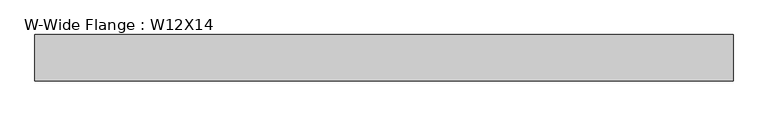
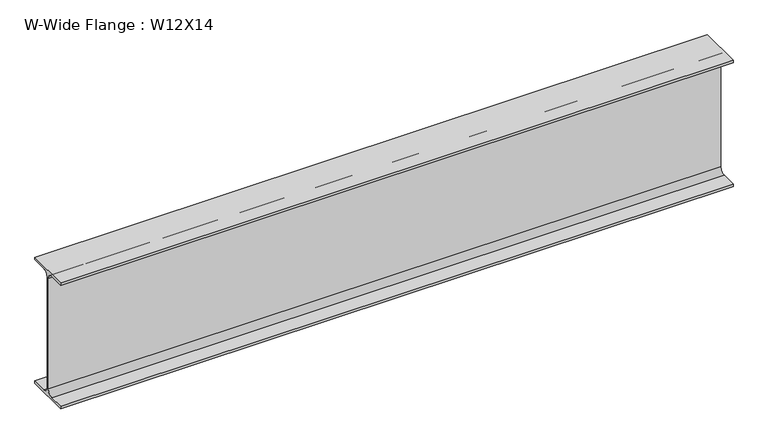
"""IFC4 building model written with IfcOpenShell, lengths in millimetres: beam geometry, W-Wide Flange : W12X14."""

from ifc_helpers import new_model, si_unit, point, frame, frame_2d, origin, place, context, project, spatial, polyline, circle_curve, trimmed, segment, composite_curve, outline, extrude, source, transform, mapped, element, save


def w_wide_flange_w12x14_438619d2(model_context):
    return source(origin(), model_context, "Body", "SweptSolid", [
        extrude(outline(composite_curve([segment(polyline([(50.419, -145.415), (50.419, -151.13), (-50.419, -151.13), (-50.419, -145.415), (-15.875, -145.415)]), True, "CONTINUOUS"), segment(trimmed(circle_curve(frame_2d((-15.875, -132.08)), 13.335), [point((-15.875, -145.415))], [point((-2.54, -132.08))], True, "CARTESIAN"), True, "CONTINUOUS"), segment(polyline([(-2.54, -132.08), (-2.54, 132.08)]), True, "CONTINUOUS"), segment(trimmed(circle_curve(frame_2d((-15.875, 132.08)), 13.335), [point((-2.54, 132.08))], [point((-15.875, 145.415))], True, "CARTESIAN"), True, "CONTINUOUS"), segment(polyline([(-15.875, 145.415), (-50.419, 145.415), (-50.419, 151.13), (50.419, 151.13), (50.419, 145.415), (15.875, 145.415)]), True, "CONTINUOUS"), segment(trimmed(circle_curve(frame_2d((15.875, 132.08)), 13.335), [point((15.875, 145.415))], [point((2.54, 132.08))], True, "CARTESIAN"), True, "CONTINUOUS"), segment(polyline([(2.54, 132.08), (2.54, -132.08)]), True, "CONTINUOUS"), segment(trimmed(circle_curve(frame_2d((15.875, -132.08)), 13.335), [point((2.54, -132.08))], [point((15.875, -145.415))], True, "CARTESIAN"), True, "CONTINUOUS"), segment(polyline([(15.875, -145.415), (50.419, -145.415)]), True, "CONTINUOUS")], self_intersect=False)), frame((-762.0, 0.0, 0.0), z_axis=(1.0, 0.0, 0.0), x_axis=(0.0, 1.0, 0.0)), (0.0, 0.0, 1.0), 1524.0),
    ])


if __name__ == "__main__":
    model = new_model("IFC4")
    model_context = context("Model", 3, world=origin())
    ifc_project = project(units=[si_unit("LENGTHUNIT", "METRE", prefix="MILLI")], contexts=[model_context])
    site = spatial("IfcSite", under=ifc_project)
    building = spatial("IfcBuilding", under=site)
    placement = place(None, origin())
    w_wide_flange_w12x14_shape = w_wide_flange_w12x14_438619d2(model_context)
    element("IfcBeam", 1, ObjectType="W-Wide Flange : W12X14", at=placement, inside=building, context=model_context, shape_type="MappedRepresentation", body=[
        mapped(w_wide_flange_w12x14_shape, transform((0.0, 0.0, 0.0), x_axis=(1.0, 0.0, 0.0), y_axis=(0.0, 1.0, 0.0), z_axis=(0.0, 0.0, 1.0))),
    ])
    save(model, "model.ifc")

# Revit data of these elements
# Type "W-Wide Flange : W12X14"
#   Assembly Code = "B10"
#   W = 14
#   Length [instance default] = 5' - 0"
#   bf = 0' - 3.97"
#   d = 0' - 11.9"
#   k = 0' - 0 3/4"
#   k2 = 0' - 0.525"
#   tf = 0' - 0.225"
#   tw = 0' - 0.2"
#   A = 0.0288889 SF
#   Structural Material [instance default] = Steel ASTM A992
# Element 1 (IfcBeam, "W-Wide Flange : W12X14")
#   Materials on its faces: "Steel ASTM A992"
# Materials
#   "Steel ASTM A992": class "Metal", colour RGB 199 199 199, transparency 0, Description = "Structural steel 50ksi", Cost = 0
